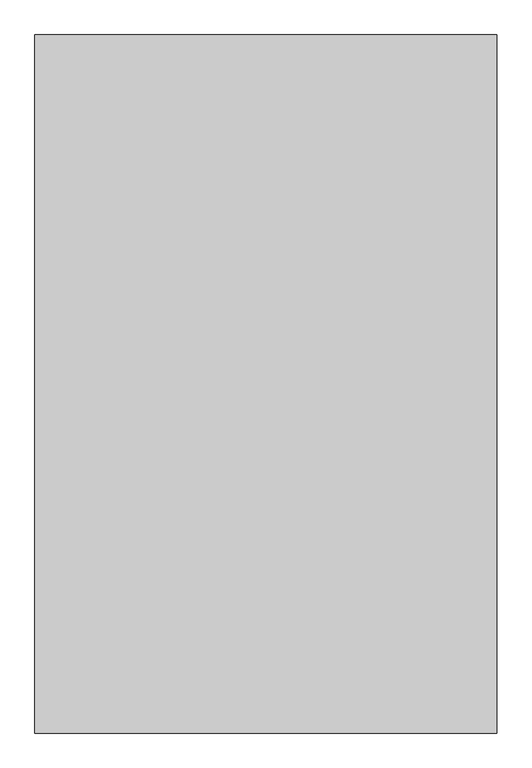
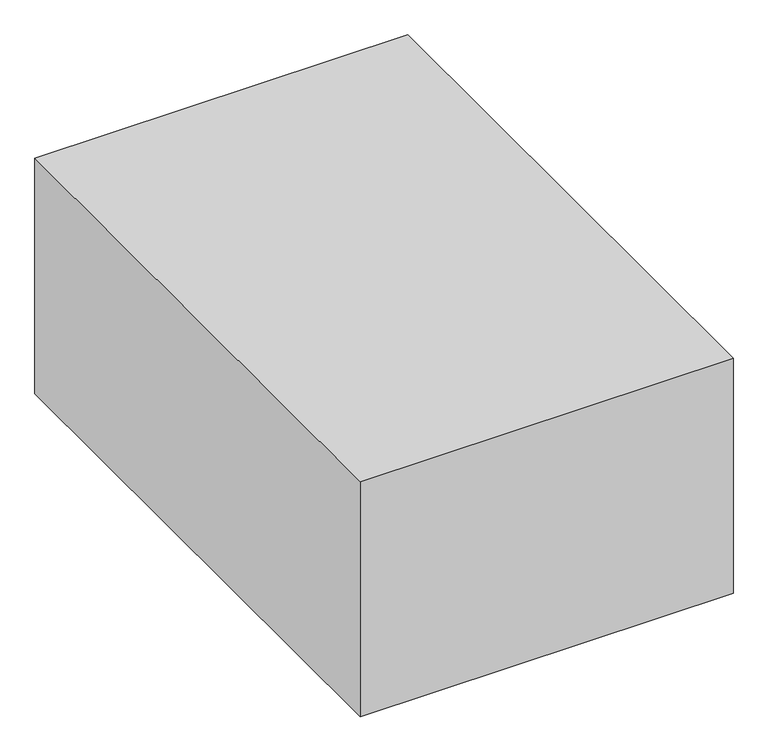
"""IFC4 building model written with IfcOpenShell, lengths in millimetres: proxy geometry, Space Planning Box_hec : Space Planning Box_hec."""

import ifcopenshell
import ifcopenshell.guid

model = None  # the IFC model being written
_history = None  # IfcOwnerHistory: only IFC2X3 demands one
_inside = {}  # id of a spatial element -> (the spatial element, [elements in it])
_under = {}  # id of a project, library or spatial element -> (it, [spatial elements below it])
_declared = {}  # id of a project -> (the project, [libraries it declares])
_typed = {}  # id of a type object -> (the type object, [elements of that type])
_made_of = {}  # id of a material, layer set ... -> (it, [elements and type objects made of it])


def new_model(schema):
    """Start an empty IFC model of exactly this schema.

    Asked for "IFC4X3", IfcOpenShell would pick the latest addendum, in which some entities
    have other attributes; the version numbers below select the first issue.
    IFC2X3 requires an IfcOwnerHistory on every rooted entity: one is made here for all.
    """
    global model, _history
    if schema == "IFC4X3":
        model = ifcopenshell.file(schema_version=(4, 3, 0, 0))
    else:
        model = ifcopenshell.file(schema=schema)
    _inside.clear()
    _under.clear()
    _declared.clear()
    _typed.clear()
    _made_of.clear()
    _history = None
    if model.schema == "IFC2X3":
        org = make("IfcOrganization", Name="unknown")
        user = make(
            "IfcPersonAndOrganization",
            ThePerson=make("IfcPerson", FamilyName="unknown"),
            TheOrganization=org,
        )
        app = make(
            "IfcApplication",
            ApplicationDeveloper=org,
            Version="unknown",
            ApplicationFullName="unknown",
            ApplicationIdentifier="unknown",
        )
        _history = make(
            "IfcOwnerHistory",
            OwningUser=user,
            OwningApplication=app,
            ChangeAction="ADDED",
            CreationDate=0,
        )
    return model


def make(cls, **values):
    """One entity of the class cls with the attributes given. An attribute that is None is left unset."""
    return model.create_entity(
        cls, **{name: value for name, value in values.items() if value is not None}
    )


def rooted(cls, **values):
    """An entity with a GlobalId (a new one), such as an element, a storey or a relation."""
    return make(cls, GlobalId=ifcopenshell.guid.new(), OwnerHistory=_history, **values)


def si_unit(unit_type, name, prefix=None):
    """IfcSIUnit, for example si_unit("LENGTHUNIT", "METRE", prefix="MILLI")."""
    return make("IfcSIUnit", UnitType=unit_type, Prefix=prefix, Name=name)


def assignment(units):
    """IfcUnitAssignment: the units of a project."""
    return None if units is None else make("IfcUnitAssignment", Units=units)


def point(xyz):
    """IfcCartesianPoint."""
    return None if xyz is None else make("IfcCartesianPoint", Coordinates=xyz)


def direction(xyz):
    """IfcDirection."""
    return None if xyz is None else make("IfcDirection", DirectionRatios=xyz)


def frame(location, z_axis=None, x_axis=None):
    """IfcAxis2Placement3D, a coordinate frame: its origin and axes. An axis left out is left unset."""
    return make(
        "IfcAxis2Placement3D",
        Location=point(location),
        Axis=direction(z_axis),
        RefDirection=direction(x_axis),
    )


def origin():
    """The frame at (0, 0, 0) with its axes left unset."""
    return frame((0.0, 0.0, 0.0))


def origin_with_axes():
    """The frame at (0, 0, 0) with the z axis (0, 0, 1) and the x axis (1, 0, 0) written out."""
    return frame((0.0, 0.0, 0.0), z_axis=(0.0, 0.0, 1.0), x_axis=(1.0, 0.0, 0.0))


def place(relative_to, where):
    """IfcLocalPlacement: puts the frame where relative to a parent placement (None: the world)."""
    return make(
        "IfcLocalPlacement", PlacementRelTo=relative_to, RelativePlacement=where
    )


def context(
    kind, dimensions, precision=None, world=None, true_north=None, identifier=None
):
    """IfcGeometricRepresentationContext, for example the 3D "Model" context."""
    return make(
        "IfcGeometricRepresentationContext",
        ContextIdentifier=identifier,
        ContextType=kind,
        CoordinateSpaceDimension=dimensions,
        Precision=precision,
        WorldCoordinateSystem=world,
        TrueNorth=true_north,
    )


def project(units=None, contexts=None):
    """IfcProject with its units and contexts."""
    return rooted(
        "IfcProject",
        Name="project",
        RepresentationContexts=contexts,
        UnitsInContext=assignment(units),
    )


def spatial(cls, under=None, at=None, **own):
    """A site, building, storey or space (cls), placed at a placement, below another one or the project."""
    s = rooted(cls, ObjectPlacement=at, **own)
    if under is not None:
        _under.setdefault(under.id(), (under, []))[1].append(s)
    return s


def polyline(points):
    """IfcPolyline through the points."""
    return make("IfcPolyline", Points=[point(p) for p in points])


def outline(outer, holes=None, kind="AREA"):
    """IfcArbitraryClosedProfileDef: a profile drawn as a closed curve; with holes, ...WithVoids."""
    if holes is None:
        return make("IfcArbitraryClosedProfileDef", ProfileType=kind, OuterCurve=outer)
    return make(
        "IfcArbitraryProfileDefWithVoids",
        ProfileType=kind,
        OuterCurve=outer,
        InnerCurves=holes,
    )


def extrude(swept, where, along, depth):
    """IfcExtrudedAreaSolid: the profile swept, set in the frame where, extruded along a direction by depth."""
    return make(
        "IfcExtrudedAreaSolid",
        SweptArea=swept,
        Position=where,
        ExtrudedDirection=direction(along),
        Depth=depth,
    )


def shape(context_of_items, identifier, shape_type, items):
    """IfcShapeRepresentation: the items that make up one representation, for example the "Body"."""
    return make(
        "IfcShapeRepresentation",
        ContextOfItems=context_of_items,
        RepresentationIdentifier=identifier,
        RepresentationType=shape_type,
        Items=items,
    )


def source(mapping_origin, context_of_items, identifier, shape_type, items):
    """IfcRepresentationMap: a shape defined once, which mapped items show again and again."""
    return make(
        "IfcRepresentationMap",
        MappingOrigin=mapping_origin,
        MappedRepresentation=shape(context_of_items, identifier, shape_type, items),
    )


def transform(
    local_origin,
    x_axis=None,
    y_axis=None,
    z_axis=None,
    scale=None,
    scale2=None,
    scale3=None,
    uniform=True,
):
    """IfcCartesianTransformationOperator3D, or its non-uniform kind. x_axis, y_axis, z_axis: its Axis1, 2, 3."""
    if uniform:
        return make(
            "IfcCartesianTransformationOperator3D",
            Axis1=direction(x_axis),
            Axis2=direction(y_axis),
            LocalOrigin=point(local_origin),
            Scale=scale,
            Axis3=direction(z_axis),
        )
    return make(
        "IfcCartesianTransformationOperator3DnonUniform",
        Axis1=direction(x_axis),
        Axis2=direction(y_axis),
        LocalOrigin=point(local_origin),
        Scale=scale,
        Axis3=direction(z_axis),
        Scale2=scale2,
        Scale3=scale3,
    )


def mapped(mapping_source, mapping_target):
    """IfcMappedItem: shows the shape of a source again, moved by a transform."""
    return make(
        "IfcMappedItem", MappingSource=mapping_source, MappingTarget=mapping_target
    )


def made_of(thing, what):
    """Note that an element or type object is made of a material, layer set ...; save() writes the relation."""
    if what is not None:
        _made_of.setdefault(what.id(), (what, []))[1].append(thing)
    return thing


def element(
    cls,
    number,
    at=None,
    inside=None,
    cuts=None,
    type_object=None,
    material=None,
    context=None,
    identifier="Body",
    shape_type=None,
    held_by="IfcProductDefinitionShape",
    body=None,
    shapes=None,
    **own,
):
    """One element of the class cls, such as IfcWall. Its Tag is "e" and its number.

    at: its placement. inside: the storey or other place that contains it. cuts: it is an
    opening in that element (IfcRelVoidsElement). A single representation is given by context,
    identifier, shape_type and body (its items); several are given by shapes. held_by: the class
    of the entity that holds the representations. save() writes the other relations.
    """
    e = rooted(cls, Tag="e%d" % number, ObjectPlacement=at, **own)
    if body is not None:
        shapes = [shape(context, identifier, shape_type, body)]
    if shapes is not None:
        e.Representation = make(held_by, Representations=shapes)
    if inside is not None:
        _inside.setdefault(inside.id(), (inside, []))[1].append(e)
    if cuts is not None:
        rooted(
            "IfcRelVoidsElement", RelatingBuildingElement=cuts, RelatedOpeningElement=e
        )
    if type_object is not None:
        _typed.setdefault(type_object.id(), (type_object, []))[1].append(e)
    return made_of(e, material)


def aggregate(whole, parts):
    """IfcRelAggregates: a whole, such as a stair, and the parts it consists of."""
    return rooted("IfcRelAggregates", RelatingObject=whole, RelatedObjects=parts)


def save(model, path):
    """Write the relations noted so far, then the file.

    IfcRelAggregates (storeys below a building ...), IfcRelContainedInSpatialStructure (elements
    in a storey), IfcRelDefinesByType, IfcRelAssociatesMaterial and IfcRelDeclares: one each for
    every whole, place, type object, material and project.
    """
    for whole, parts in _under.values():
        aggregate(whole, parts)
    for where, things in _inside.values():
        rooted(
            "IfcRelContainedInSpatialStructure",
            RelatedElements=things,
            RelatingStructure=where,
        )
    for kind, things in _typed.values():
        rooted("IfcRelDefinesByType", RelatedObjects=things, RelatingType=kind)
    for what, things in _made_of.values():
        rooted("IfcRelAssociatesMaterial", RelatedObjects=things, RelatingMaterial=what)
    for by, libraries in _declared.values():
        rooted("IfcRelDeclares", RelatingContext=by, RelatedDefinitions=libraries)
    model.write(path)


def generic_models_af0009da(model_context):
    return source(origin(), model_context, "Body", "SweptSolid", [
        extrude(outline(polyline([(4500.0, 6800.0), (4500.0, -6800.0), (-4500.0, -6800.0), (-4500.0, 6800.0), (4500.0, 6800.0)])), origin_with_axes(), (0.0, 0.0, 1.0), 6000.0),
    ])


if __name__ == "__main__":
    model = new_model("IFC4")
    model_context = context("Model", 3, world=origin())
    ifc_project = project(units=[si_unit("LENGTHUNIT", "METRE", prefix="MILLI")], contexts=[model_context])
    site = spatial("IfcSite", under=ifc_project)
    building = spatial("IfcBuilding", under=site)
    placement = place(None, origin())
    generic_models_shape = generic_models_af0009da(model_context)
    element("IfcBuildingElementProxy", 1, Name="Space Planning Box_hec : Space Planning Box_hec", ObjectType="Space Planning Box_hec : Space Planning Box_hec", at=placement, inside=building, context=model_context, shape_type="MappedRepresentation", body=[
        mapped(generic_models_shape, transform((0.0, 0.0, 0.0), x_axis=(1.0, 0.0, 0.0), y_axis=(0.0, 1.0, 0.0), z_axis=(0.0, 0.0, 1.0))),
    ])
    save(model, "model.ifc")

# Revit data of these elements
# Type "Space Planning Box_hec : Space Planning Box_hec"
#   Type Comments = "..."
#   Room Name [instance default] = "?"
#   Interior Finish [instance default] = ""
#   Exterior Finish [instance default] = ""
#   Department [instance default] = ""
#   Assembly Code = "..."
#   Width [instance default] = 1524 mm
#   Program Area [instance default] = 0 m²
#   Length [instance default] = 1524 mm
#   Height [instance default] = 1524 mm
#   Area [instance default] = 2.32258 m²
#   Fill Color [instance default] = Cyan
#   Default Elevation = 0
# Element 1 (IfcBuildingElementProxy, "Space Planning Box_hec : Space Planning Box_hec")
#   Room Name = "Engineer Room"
#   Interior Finish = "IF3"
#   Exterior Finish = "EF1"
#   Department = "CI"
#   Width = 9000 mm
#   Program Area = 120 m²
#   Length = 13600 mm
#   Height = 6000 mm
#   Area = 122.4 m²
#   Fill Color = Lime
#   Materials on its faces: "Lime"
# Materials
#   "Cyan": class "Generic", colour RGB 0 255 255, transparency 0.2, Cost = 0
#   "Lime": class "Generic", colour RGB 0 255 0, transparency 0.2, Cost = 0
